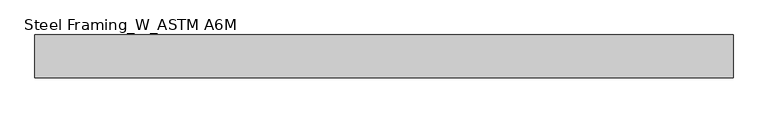
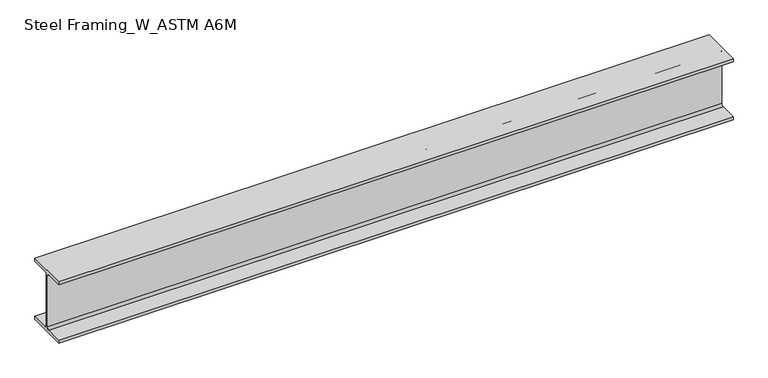
"""IFC4 building model written with IfcOpenShell, lengths in millimetres: beam geometry, Steel Framing_W_ASTM A6M : H_SB_AR_S02_W200x31.3_B6."""

from ifc_helpers import new_model, si_unit, point, frame, frame_2d, origin, place, context, project, spatial, polyline, circle_curve, trimmed, segment, composite_curve, outline, extrude, source, transform, mapped, element, save


def steel_framing_w_astm_a6m_1b426b15(model_context):
    return source(origin(), model_context, "Body", "SweptSolid", [
        extrude(outline(composite_curve([segment(polyline([(67.0, -94.8), (67.0, -105.0), (-67.0, -105.0), (-67.0, -94.8), (-10.775, -94.8)]), True, "CONTINUOUS"), segment(trimmed(circle_curve(frame_2d((-10.775, -87.2)), 7.6), [point((-10.775, -94.8))], [point((-3.175, -87.2))], True, "CARTESIAN"), True, "CONTINUOUS"), segment(polyline([(-3.175, -87.2), (-3.175, 87.2)]), True, "CONTINUOUS"), segment(trimmed(circle_curve(frame_2d((-10.775, 87.2)), 7.6), [point((-3.175, 87.2))], [point((-10.775, 94.8))], True, "CARTESIAN"), True, "CONTINUOUS"), segment(polyline([(-10.775, 94.8), (-67.0, 94.8), (-67.0, 105.0), (67.0, 105.0), (67.0, 94.8), (10.775, 94.8)]), True, "CONTINUOUS"), segment(trimmed(circle_curve(frame_2d((10.775, 87.2)), 7.6), [point((10.775, 94.8))], [point((3.175, 87.2))], True, "CARTESIAN"), True, "CONTINUOUS"), segment(polyline([(3.175, 87.2), (3.175, -87.2)]), True, "CONTINUOUS"), segment(trimmed(circle_curve(frame_2d((10.775, -87.2)), 7.6), [point((3.175, -87.2))], [point((10.775, -94.8))], True, "CARTESIAN"), True, "CONTINUOUS"), segment(polyline([(10.775, -94.8), (67.0, -94.8)]), True, "CONTINUOUS")], self_intersect=False)), frame((-1135.8, 0.0, 0.0), z_axis=(1.0, 0.0, 0.0), x_axis=(0.0, 1.0, 0.0)), (0.0, 0.0, 1.0), 2189.1),
    ])


if __name__ == "__main__":
    model = new_model("IFC4")
    model_context = context("Model", 3, world=origin())
    ifc_project = project(units=[si_unit("LENGTHUNIT", "METRE", prefix="MILLI")], contexts=[model_context])
    site = spatial("IfcSite", under=ifc_project)
    building = spatial("IfcBuilding", under=site)
    placement = place(None, origin())
    steel_framing_w_astm_a6m_shape = steel_framing_w_astm_a6m_1b426b15(model_context)
    element("IfcBeam", 1, ObjectType="Steel Framing_W_ASTM A6M : H_SB_AR_S02_W200x31.3_B6", at=placement, inside=building, context=model_context, shape_type="MappedRepresentation", body=[
        mapped(steel_framing_w_astm_a6m_shape, transform((0.0, 0.0, 0.0), x_axis=(1.0, 0.0, 0.0), y_axis=(0.0, 1.0, 0.0), z_axis=(0.0, 0.0, 1.0))),
    ])
    save(model, "model.ifc")

# Revit data of these elements
# Type "Steel Framing_W_ASTM A6M : H_SB_AR_S02_W200x31.3_B6"
#   Type Mark = "B6"
#   Section Name Key = "W8x21"
#   Width = 13.4 cm
#   Web Thickness = 0.635 cm
#   Web Fillet = 0.76 cm
#   Warping Constant = 40800.0 cm⁶
#   Torsional Moment of Inertia = 11.70 cm⁴
#   Section Area = 39.7 cm²
#   Plastic Modulus weak axis = 93.2 cm³
#   Plastic Modulus strong axis = 334.0 cm³
#   Perimeter = 0.93 m²/m
#   Nominal Weight = 31.30 kgf/m
#   Moment of Inertia weak axis = 407.00 cm⁴
#   Moment of Inertia strong axis = 3130.00 cm⁴
#   Height = 21.0 cm
#   Flange Thickness = 1.02 cm
#   Elastic Modulus weak axis = 60.8 cm³
#   Elastic Modulus strong axis = 298.0 cm³
#   Centroid Vertical = 10.5 cm
#   Centroid Horizontal = 6.7 cm
#   Length [instance default] = 1500 mm
#   Structural Material [instance default] = Steel, 45-345
#   Bolt Spacing = 0
#   Assembly Code = ""
# Element 1 (IfcBeam, "Steel Framing_W_ASTM A6M : H_SB_AR_S02_W200x31.3_B6")
#   Materials on its faces: "Steel, 45-345"
# Materials
#   "Steel, 45-345": class "Metal", colour RGB 189 187 185, transparency 0, Description = "Steel 345 MPa", Cost = 0
